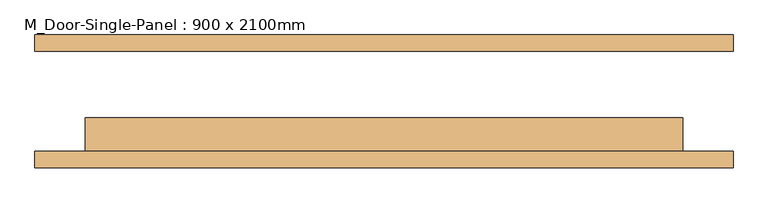
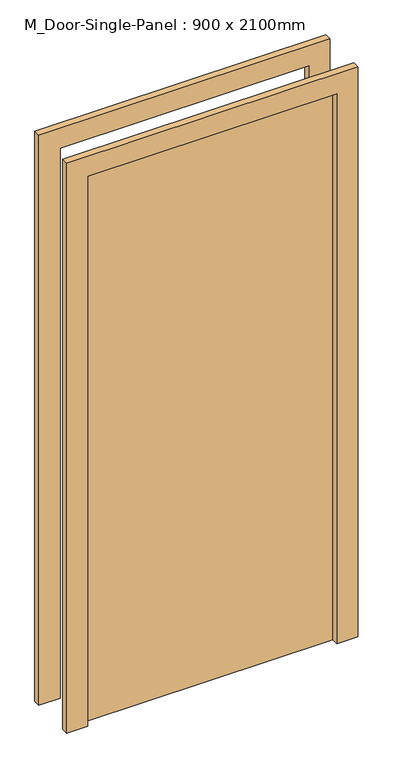
"""IFC4 building model written with IfcOpenShell, lengths in millimetres: door geometry, M_Door-Single-Panel : 900 x 2100mm."""

from ifc_helpers import new_model, si_unit, frame, origin, origin_with_axes, place, context, project, spatial, polyline, outline, extrude, source, transform, mapped, element, save


def m_door_single_panel_900_x_2100mm_e2860c58(model_context):
    return source(origin(), model_context, "Body", "SweptSolid", [
        extrude(outline(polyline([(450.0, -25.0), (450.0, -75.0), (-450.0, -75.0), (-450.0, -25.0), (450.0, -25.0)])), origin_with_axes(), (0.0, 0.0, 1.0), 2100.0),
        extrude(outline(polyline([(2176.2, 526.2), (2176.2, -526.2), (0.0, -526.2), (0.0, -450.0), (2100.0, -450.0), (2100.0, 450.0), (0.0, 450.0), (0.0, 526.2), (2176.2, 526.2)])), frame((0.0, 75.0, 0.0), z_axis=(0.0, 1.0, 0.0), x_axis=(0.0, 0.0, 1.0)), (0.0, 0.0, 1.0), 25.0),
        extrude(outline(polyline([(2176.2, -526.2), (0.0, -526.2), (0.0, -450.0), (2100.0, -450.0), (2100.0, 450.0), (0.0, 450.0), (0.0, 526.2), (2176.2, 526.2), (2176.2, -526.2)])), frame((0.0, -100.0, 0.0), z_axis=(0.0, 1.0, 0.0), x_axis=(0.0, 0.0, 1.0)), (0.0, 0.0, 1.0), 25.0),
    ])


if __name__ == "__main__":
    model = new_model("IFC4")
    model_context = context("Model", 3, world=origin())
    ifc_project = project(units=[si_unit("LENGTHUNIT", "METRE", prefix="MILLI")], contexts=[model_context])
    site = spatial("IfcSite", under=ifc_project)
    building = spatial("IfcBuilding", under=site)
    placement = place(None, origin())
    m_door_single_panel_900_x_2100mm_shape = m_door_single_panel_900_x_2100mm_e2860c58(model_context)
    element("IfcDoor", 1, ObjectType="M_Door-Single-Panel : 900 x 2100mm", at=placement, inside=building, context=model_context, shape_type="MappedRepresentation", body=[
        mapped(m_door_single_panel_900_x_2100mm_shape, transform((0.0, 0.0, 0.0), x_axis=(1.0, 0.0, 0.0), y_axis=(0.0, 1.0, 0.0), z_axis=(0.0, 0.0, 1.0))),
    ])
    save(model, "model.ifc")

# Revit data of these elements
# Type "M_Door-Single-Panel : 900 x 2100mm"
#   Type Mark = "48"
#   Construction Type Id = "DOOR"
#   Analytic Construction = "Wooden"
#   Thickness = 0.05 m
#   Thermal Resistance (R) = 0.455703 (m²·K)/W
#   Swing Angle [instance default] = 90.00°
#   Heat Transfer Coefficient (U) = 2.19465 W/(m²·K)
#   Height = 2.10 m
#   Trim Projection Ext = 0.025 m
#   Trim Projection Int = 0.025 m
#   Trim Width = 0.08 m
#   Width = 0.90 m
#   Define Thermal Properties by = 1
#   Panel Material = Wood - Birch - Solid Stained Light Low Gloss
#   Trim Material = Paint - Sienna
#   Visual Light Transmittance = 0
#   Solar Heat Gain Coefficient = 0
#   Function = (empty or 0)
#   Wall Closure = (empty or 0)
# Element 1 (IfcDoor, "M_Door-Single-Panel : 900 x 2100mm")
#   Materials on its faces: "Paint - Sienna", "Wood - Birch - Solid Stained Light Low Gloss"
# Materials
#   "Wood - Birch - Solid Stained Light Low Gloss": class "Wood", colour RGB 210 159 95, transparency 0, Cost = 0
#   "Paint - Sienna": class "Miscellaneous", colour RGB 118 70 51, transparency 0, Cost = 0
